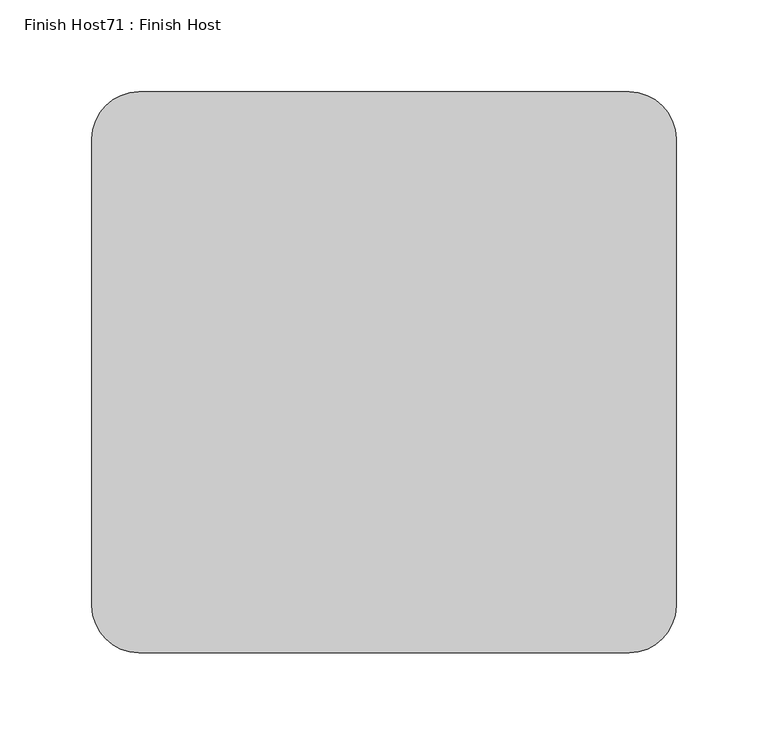
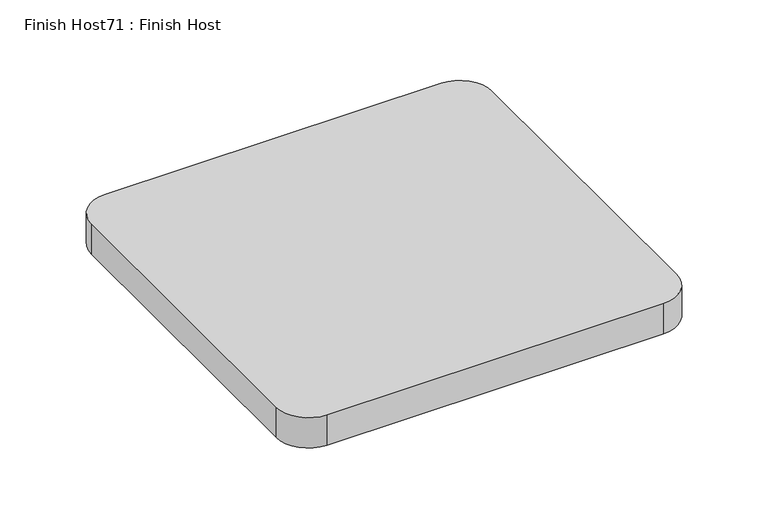
"""IFC4 building model written with IfcOpenShell, lengths in millimetres: proxy geometry, Finish Host71 : Finish Host."""

from ifc_helpers import new_model, si_unit, point, frame_2d, origin, origin_with_axes, place, context, project, spatial, polyline, circle_curve, trimmed, segment, composite_curve, outline, extrude, source, transform, mapped, element, save


def finish_host71_finish_host_a2c4ce34(model_context):
    return source(origin(), model_context, "Body", "SweptSolid", [
        extrude(outline(composite_curve([segment(polyline([(-17113.2939795, 9121.5610533), (-17113.2939795, 9375.5610533)]), True, "CONTINUOUS"), segment(trimmed(circle_curve(frame_2d((-17087.8939795, 9375.5610533)), 25.4), [point((-17113.2939795, 9375.5610533))], [point((-17087.8939795, 9400.9610533))], False, "CARTESIAN"), True, "CONTINUOUS"), segment(polyline([(-17087.8939795, 9400.9610533), (-16821.1939795, 9400.9610533)]), True, "CONTINUOUS"), segment(trimmed(circle_curve(frame_2d((-16821.1939795, 9375.5610533)), 25.4), [point((-16821.1939795, 9400.9610533))], [point((-16795.7939795, 9375.5610533))], False, "CARTESIAN"), True, "CONTINUOUS"), segment(polyline([(-16795.7939795, 9375.5610533), (-16795.7939795, 9121.5610533)]), True, "CONTINUOUS"), segment(trimmed(circle_curve(frame_2d((-16821.1939795, 9121.5610533)), 25.4), [point((-16795.7939795, 9121.5610533))], [point((-16821.1939795, 9096.1610533))], False, "CARTESIAN"), True, "CONTINUOUS"), segment(polyline([(-16821.1939795, 9096.1610533), (-17087.8939795, 9096.1610533)]), True, "CONTINUOUS"), segment(trimmed(circle_curve(frame_2d((-17087.8939795, 9121.5610533)), 25.4), [point((-17087.8939795, 9096.1610533))], [point((-17113.2939795, 9121.5610533))], False, "CARTESIAN"), True, "CONTINUOUS")], self_intersect=False)), origin_with_axes(), (0.0, 0.0, 1.0), 25.4),
    ])


if __name__ == "__main__":
    model = new_model("IFC4")
    model_context = context("Model", 3, world=origin())
    ifc_project = project(units=[si_unit("LENGTHUNIT", "METRE", prefix="MILLI")], contexts=[model_context])
    site = spatial("IfcSite", under=ifc_project)
    building = spatial("IfcBuilding", under=site)
    placement = place(None, origin())
    finish_host71_finish_host_shape = finish_host71_finish_host_a2c4ce34(model_context)
    element("IfcBuildingElementProxy", 1, Name="Finish Host71 : Finish Host", ObjectType="Finish Host71 : Finish Host", at=placement, inside=building, context=model_context, shape_type="MappedRepresentation", body=[
        mapped(finish_host71_finish_host_shape, transform((0.0, 0.0, 0.0), x_axis=(1.0, 0.0, 0.0), y_axis=(0.0, 1.0, 0.0), z_axis=(0.0, 0.0, 1.0))),
    ])
    save(model, "model.ifc")

# Revit data of these elements
# Type "Finish Host71 : Finish Host"
#   Countertop Material = Glass - Teknion - A5 - Standard - Clear
# Element 1 (IfcBuildingElementProxy, "Finish Host71 : Finish Host")
#   Materials on its faces: "Glass - Teknion - A5 - Standard - Clear"
# Materials
#   "Glass - Teknion - A5 - Standard - Clear": class "Glass", colour RGB 221 221 221, transparency 0.95, Model = "A5", Manufacturer = "Teknion Studio", URL = "http://www.teknion.com/", Description = "Clear", Cost = 0
